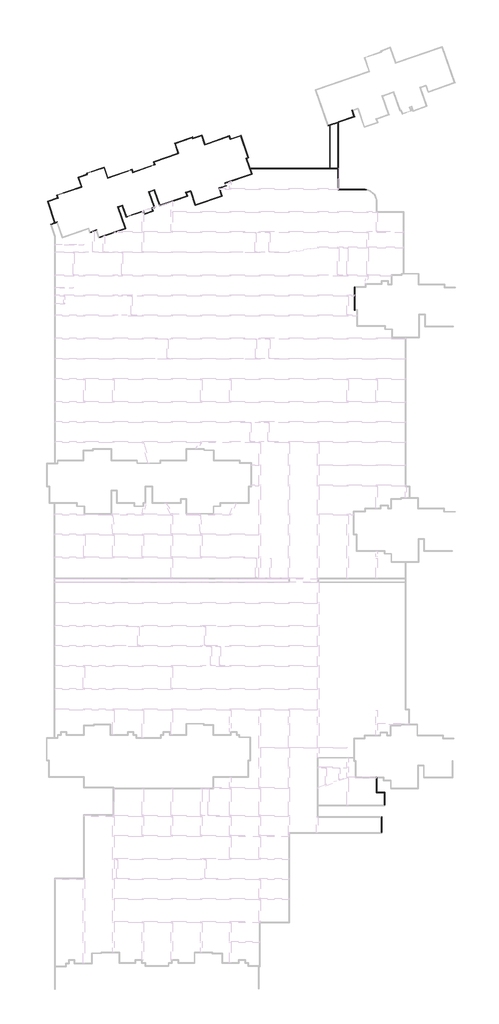
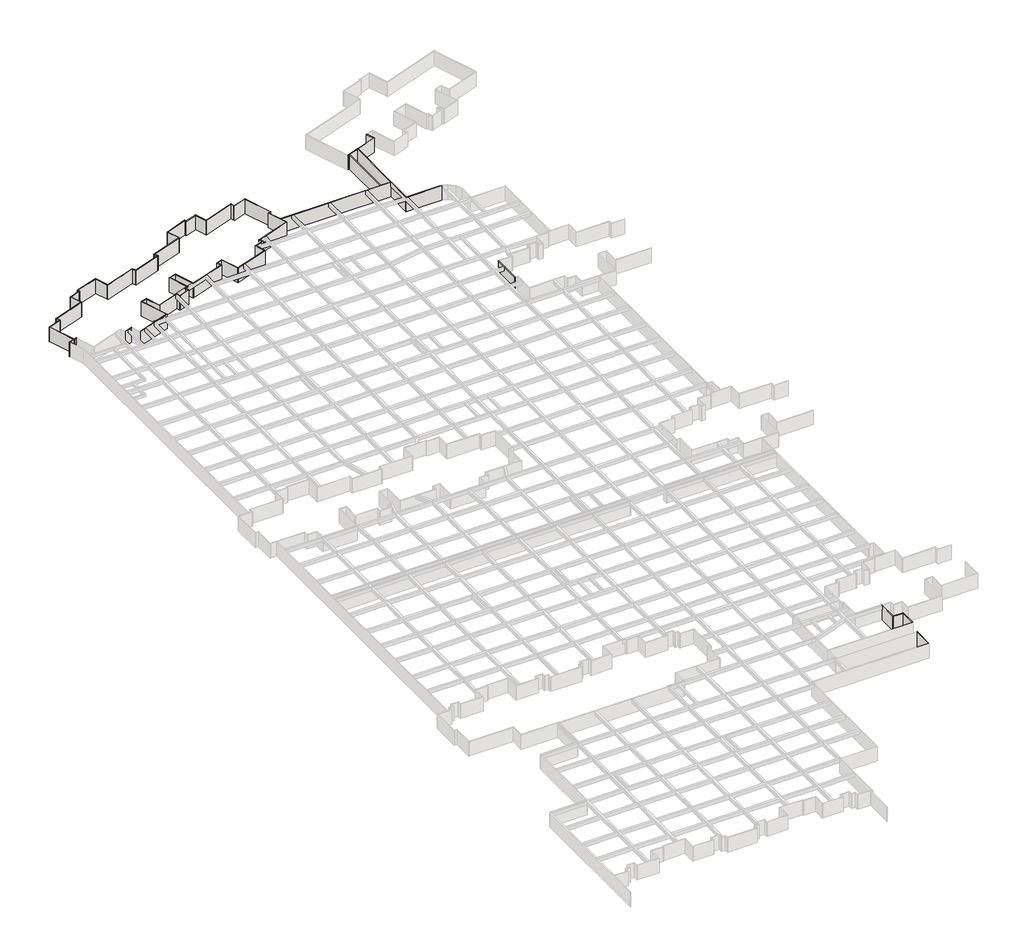
# One storey, part 4 of 14: 62 walls.
"""IFC4 building model written with IfcOpenShell, lengths in millimetres."""

from ifc_helpers import new_model, si_unit, origin, place, context, project, spatial, faceted_brep, element, save

model = new_model("IFC4")

# Units and contexts
model_context = context("Model", 3, world=origin())
ifc_project = project(units=[si_unit("LENGTHUNIT", "METRE", prefix="MILLI")], contexts=[model_context])

# Site, building, storey
site = spatial("IfcSite", under=ifc_project)
building = spatial("IfcBuilding", under=site)
storey = spatial("IfcBuildingStorey", under=building, Name="户型图", Elevation=0.0)

# Walls
placement = place(None, origin())
element("IfcWall", 1, ObjectType="所有墙体", at=placement, inside=storey, context=model_context, shape_type="Brep", body=[
    faceted_brep([(-587687.3228237, -18726.1128295, 0.0), (-586876.8743145, -21142.8199356, 0.0), (-586838.7202272, -21256.5930536, 0.0), (-586838.7202272, -21256.5930536, 3300.0), (-586876.8743145, -21142.8199356, 3300.0), (-587687.3228237, -18726.1128295, 3300.0), (-587575.1897502, -18683.0689754, 0.0), (-587575.1897502, -18683.0689754, 3300.0), (-586725.0230806, -21218.2131681, 3300.0), (-586725.0230806, -21218.2131681, 0.0)], [[[0, 1, 2, 3, 4, 5]], [[6, 7, 8, 9]], [[2, 1, 0, 6, 9]], [[5, 4, 3, 8, 7]], [[3, 2, 9, 8]], [[0, 5, 7, 6]]]),
])
element("IfcWall", 2, ObjectType="所有墙体", at=placement, inside=storey, context=model_context, shape_type="Brep", body=[
    faceted_brep([(-586876.8743145, -21142.8199356, 0.0), (-593604.0549797, -23413.6634153, 0.0), (-593604.0549797, -23413.6634153, 3300.0), (-586876.8743145, -21142.8199356, 3300.0), (-586838.7202272, -21256.5930536, 0.0), (-586838.7202272, -21256.5930536, 3300.0), (-593451.9782472, -23488.9805279, 3300.0), (-593565.6751698, -23527.3603378, 3300.0), (-593565.6751698, -23527.3603378, 0.0), (-593451.9782472, -23488.9805279, 0.0)], [[[0, 1, 2, 3]], [[4, 5, 6, 7, 8, 9]], [[1, 0, 4, 9, 8]], [[3, 2, 7, 6, 5]], [[0, 3, 5, 4]], [[2, 1, 8, 7]]]),
])
element("IfcWall", 3, ObjectType="所有墙体", at=placement, inside=storey, context=model_context, shape_type="Brep", body=[
    faceted_brep([(-593565.6751698, -23527.3603378, 0.0), (-593332.1963521, -24219.021477, 0.0), (-593293.8165422, -24332.7183995, 0.0), (-593293.8165422, -24332.7183995, 3300.0), (-593332.1963521, -24219.021477, 3300.0), (-593565.6751698, -23527.3603378, 3300.0), (-593451.9782472, -23488.9805279, 0.0), (-593451.9782472, -23488.9805279, 3300.0), (-593180.1196197, -24294.3385896, 3300.0), (-593180.1196197, -24294.3385896, 0.0)], [[[0, 1, 2, 3, 4, 5]], [[6, 7, 8, 9]], [[2, 1, 0, 6, 9]], [[5, 4, 3, 8, 7]], [[0, 5, 7, 6]], [[3, 2, 9, 8]]]),
])
element("IfcWall", 4, ObjectType="所有墙体", at=placement, inside=storey, context=model_context, shape_type="Brep", body=[
    faceted_brep([(-593332.1963521, -24219.021477, 0.0), (-596112.814503, -25157.6537082, 0.0), (-596112.814503, -25157.6537082, 3300.0), (-593332.1963521, -24219.021477, 3300.0), (-593293.8165422, -24332.7183995, 0.0), (-593293.8165422, -24332.7183995, 3300.0), (-595960.7377706, -25232.9708208, 3300.0), (-596074.4346931, -25271.3506307, 3300.0), (-596074.4346931, -25271.3506307, 0.0), (-595960.7377706, -25232.9708208, 0.0)], [[[0, 1, 2, 3]], [[4, 5, 6, 7, 8, 9]], [[1, 0, 4, 9, 8]], [[3, 2, 7, 6, 5]], [[0, 3, 5, 4]], [[2, 1, 8, 7]]]),
])
element("IfcWall", 5, ObjectType="所有墙体", at=placement, inside=storey, context=model_context, shape_type="Brep", body=[
    faceted_brep([(-596074.4346931, -25271.3506307, 0.0), (-594137.7360341, -31008.6556848, 0.0), (-594099.3942841, -31122.2398581, 0.0), (-594099.3942841, -31122.2398581, 3300.0), (-594137.7360341, -31008.6556848, 3300.0), (-596074.4346931, -25271.3506307, 3300.0), (-595960.7377706, -25232.9708208, 0.0), (-595960.7377706, -25232.9708208, 3300.0), (-594024.0010516, -30970.3886242, 3300.0), (-593985.6211661, -31084.0857708, 3300.0), (-593985.6211661, -31084.0857708, 0.0), (-594024.0010516, -30970.3886242, 0.0)], [[[0, 1, 2, 3, 4, 5]], [[6, 7, 8, 9, 10, 11]], [[2, 1, 0, 6, 11, 10]], [[5, 4, 3, 9, 8, 7]], [[0, 5, 7, 6]], [[3, 2, 10, 9]]]),
])
element("IfcWall", 6, ObjectType="所有墙体", at=placement, inside=storey, context=model_context, shape_type="Brep", body=[
    faceted_brep([(-593985.6211661, -31084.0857708, 0.0), (-593530.5298151, -30931.4697976, 0.0), (-593416.7566971, -30893.3157103, 0.0), (-593416.7566971, -30893.3157103, 3300.0), (-593530.5298151, -30931.4697976, 3300.0), (-593985.6211661, -31084.0857708, 3300.0), (-594024.0010516, -30970.3886242, 0.0), (-594024.0010516, -30970.3886242, 3300.0), (-593455.1365827, -30779.6185637, 3300.0), (-593455.1365827, -30779.6185637, 0.0)], [[[0, 1, 2, 3, 4, 5]], [[6, 7, 8, 9]], [[2, 1, 0, 6, 9]], [[5, 4, 3, 8, 7]], [[0, 5, 7, 6]], [[3, 2, 9, 8]]]),
])
element("IfcWall", 7, ObjectType="所有墙体", at=placement, inside=storey, context=model_context, shape_type="Brep", body=[
    faceted_brep([(-584459.5809867, -33672.8456024, 0.0), (-582772.9638867, -33103.5070288, 0.0), (-582659.2669642, -33065.1272189, 0.0), (-582659.2669642, -33065.1272189, 3300.0), (-582772.9638867, -33103.5070288, 3300.0), (-584459.5809867, -33672.8456024, 3300.0), (-584497.735074, -33559.0724844, 0.0), (-584497.735074, -33559.0724844, 3300.0), (-582697.6467741, -32951.4302963, 3300.0), (-582697.6467741, -32951.4302963, 0.0)], [[[0, 1, 2, 3, 4, 5]], [[6, 7, 8, 9]], [[2, 1, 0, 6, 9]], [[5, 4, 3, 8, 7]], [[0, 5, 7, 6]], [[3, 2, 9, 8]]]),
])
element("IfcWall", 8, ObjectType="所有墙体", at=placement, inside=storey, context=model_context, shape_type="Brep", body=[
    faceted_brep([(-581987.6202907, -35054.823363, 0.0), (-574770.6130433, -32618.6328334, 0.0), (-574770.6130433, -32618.6328334, 3300.0), (-581987.6202907, -35054.823363, 3300.0), (-582026.0001006, -34941.1264405, 0.0), (-582026.0001006, -34941.1264405, 3300.0), (-574922.6897757, -32543.3157207, 3300.0), (-574808.9928531, -32504.9359109, 3300.0), (-574808.9928531, -32504.9359109, 0.0), (-574922.6897757, -32543.3157207, 0.0)], [[[0, 1, 2, 3]], [[4, 5, 6, 7, 8, 9]], [[1, 0, 4, 9, 8]], [[3, 2, 7, 6, 5]], [[0, 3, 5, 4]], [[2, 1, 8, 7]]]),
])
element("IfcWall", 9, ObjectType="所有墙体", at=placement, inside=storey, context=model_context, shape_type="Brep", body=[
    faceted_brep([(-574808.9928531, -32504.9359109, 0.0), (-576769.5614763, -26696.91811, 0.0), (-576807.9412862, -26583.2211874, 0.0), (-576807.9412862, -26583.2211874, 3300.0), (-576769.5614763, -26696.91811, 3300.0), (-574808.9928531, -32504.9359109, 3300.0), (-574922.6897757, -32543.3157207, 0.0), (-574922.6897757, -32543.3157207, 3300.0), (-576921.6382087, -26621.6009973, 3300.0), (-576921.6382087, -26621.6009973, 0.0)], [[[0, 1, 2, 3, 4, 5]], [[6, 7, 8, 9]], [[2, 1, 0, 6, 9]], [[5, 4, 3, 8, 7]], [[0, 5, 7, 6]], [[3, 2, 9, 8]]]),
])
element("IfcWall", 10, ObjectType="所有墙体", at=placement, inside=storey, context=model_context, shape_type="Brep", body=[
    faceted_brep([(-576769.5614763, -26696.91811, 0.0), (-575651.541738, -26319.5166463, 0.0), (-575537.8448155, -26281.1368364, 0.0), (-575537.8448155, -26281.1368364, 3300.0), (-575651.541738, -26319.5166463, 3300.0), (-576769.5614763, -26696.91811, 3300.0), (-576807.9412862, -26583.2211874, 0.0), (-576807.9412862, -26583.2211874, 3300.0), (-575576.2246253, -26167.4399139, 3300.0), (-575576.2246253, -26167.4399139, 0.0)], [[[0, 1, 2, 3, 4, 5]], [[6, 7, 8, 9]], [[2, 1, 0, 6, 9]], [[5, 4, 3, 8, 7]], [[0, 5, 7, 6]], [[3, 2, 9, 8]]]),
])
element("IfcWall", 11, ObjectType="所有墙体", at=placement, inside=storey, context=model_context, shape_type="Brep", body=[
    faceted_brep([(-575651.541738, -26319.5166463, 0.0), (-574596.1350237, -29446.0692758, 0.0), (-574596.1350237, -29446.0692758, 3300.0), (-575651.541738, -26319.5166463, 3300.0), (-575537.8448155, -26281.1368364, 0.0), (-575537.8448155, -26281.1368364, 3300.0), (-574520.7417912, -29294.2180419, 3300.0), (-574482.3619057, -29407.9151885, 3300.0), (-574482.3619057, -29407.9151885, 0.0), (-574520.7417912, -29294.2180419, 0.0)], [[[0, 1, 2, 3]], [[4, 5, 6, 7, 8, 9]], [[1, 0, 4, 9, 8]], [[3, 2, 7, 6, 5]], [[0, 3, 5, 4]], [[2, 1, 8, 7]]]),
])
element("IfcWall", 12, ObjectType="所有墙体", at=placement, inside=storey, context=model_context, shape_type="Brep", body=[
    faceted_brep([(-574482.3619057, -29407.9151885, 0.0), (-569950.4085273, -27888.1137818, 0.0), (-569836.6354093, -27849.9596945, 0.0), (-569836.6354093, -27849.9596945, 3300.0), (-569950.4085273, -27888.1137818, 3300.0), (-574482.3619057, -29407.9151885, 3300.0), (-574520.7417912, -29294.2180419, 0.0), (-574520.7417912, -29294.2180419, 3300.0), (-569875.0152948, -27736.2625479, 3300.0), (-569875.0152948, -27736.2625479, 0.0)], [[[0, 1, 2, 3, 4, 5]], [[6, 7, 8, 9]], [[2, 1, 0, 6, 9]], [[5, 4, 3, 8, 7]], [[0, 5, 7, 6]], [[3, 2, 9, 8]]]),
])
element("IfcWall", 13, ObjectType="所有墙体", at=placement, inside=storey, context=model_context, shape_type="Brep", body=[
    faceted_brep([(-569950.4085273, -27888.1137818, 0.0), (-569694.5050683, -28646.2060146, 0.0), (-569694.5050683, -28646.2060146, 3300.0), (-569950.4085273, -27888.1137818, 3300.0), (-569836.6354093, -27849.9596945, 0.0), (-569836.6354093, -27849.9596945, 3300.0), (-569619.1879557, -28494.1292822, 3300.0), (-569580.8081458, -28607.8262047, 3300.0), (-569580.8081458, -28607.8262047, 0.0), (-569619.1879557, -28494.1292822, 0.0)], [[[0, 1, 2, 3]], [[4, 5, 6, 7, 8, 9]], [[1, 0, 4, 9, 8]], [[3, 2, 7, 6, 5]], [[0, 3, 5, 4]], [[2, 1, 8, 7]]]),
])
element("IfcWall", 14, ObjectType="所有墙体", at=placement, inside=storey, context=model_context, shape_type="Brep", body=[
    faceted_brep([(-569580.8081458, -28607.8262047, 0.0), (-567259.5995736, -27824.2733903, 0.0), (-567259.5995736, -27824.2733903, 3300.0), (-569580.8081458, -28607.8262047, 3300.0), (-569619.1879557, -28494.1292822, 0.0), (-569619.1879557, -28494.1292822, 3300.0), (-567411.4508075, -27748.8801578, 3300.0), (-567297.7536609, -27710.5002723, 3300.0), (-567297.7536609, -27710.5002723, 0.0), (-567411.4508075, -27748.8801578, 0.0)], [[[0, 1, 2, 3]], [[4, 5, 6, 7, 8, 9]], [[1, 0, 4, 9, 8]], [[3, 2, 7, 6, 5]], [[0, 3, 5, 4]], [[2, 1, 8, 7]]]),
])
element("IfcWall", 15, ObjectType="所有墙体", at=placement, inside=storey, context=model_context, shape_type="Brep", body=[
    faceted_brep([(-567297.7536609, -27710.5002723, 0.0), (-567513.9596543, -27065.7874317, 0.0), (-567552.1137415, -26952.0143137, 0.0), (-567552.1137415, -26952.0143137, 3300.0), (-567513.9596543, -27065.7874317, 3300.0), (-567297.7536609, -27710.5002723, 3300.0), (-567411.4508075, -27748.8801578, 0.0), (-567411.4508075, -27748.8801578, 3300.0), (-567665.8108881, -26990.3941992, 3300.0), (-567665.8108881, -26990.3941992, 0.0)], [[[0, 1, 2, 3, 4, 5]], [[6, 7, 8, 9]], [[2, 1, 0, 6, 9]], [[5, 4, 3, 8, 7]], [[0, 5, 7, 6]], [[3, 2, 9, 8]]]),
])
element("IfcWall", 16, ObjectType="所有墙体", at=placement, inside=storey, context=model_context, shape_type="Brep", body=[
    faceted_brep([(-567513.9596543, -27065.7874317, 0.0), (-566850.6148569, -26841.8671476, 0.0), (-566850.6148569, -26841.8671476, 2500.0), (-566850.6148569, -26841.8671476, 3300.0), (-567238.9034733, -26972.9387979, 3300.0), (-567513.9596543, -27065.7874317, 3300.0), (-567552.1137415, -26952.0143137, 0.0), (-567552.1137415, -26952.0143137, 3300.0), (-567277.2832832, -26859.2418753, 3300.0), (-567002.6915893, -26766.5500349, 3300.0), (-566888.9946667, -26728.170225, 3300.0), (-566888.9946667, -26728.170225, 0.0), (-567002.6915893, -26766.5500349, 0.0)], [[[0, 1, 2, 3, 4, 5]], [[6, 7, 8, 9, 10, 11, 12]], [[1, 0, 6, 12, 11]], [[5, 4, 3, 10, 9, 8, 7]], [[0, 5, 7, 6]], [[3, 2, 1, 11, 10]]]),
])
element("IfcWall", 17, ObjectType="所有墙体", at=placement, inside=storey, context=model_context, shape_type="Brep", body=[
    faceted_brep([(-566888.9946667, -26728.170225, 0.0), (-568292.9695403, -22569.0140692, 0.0), (-568331.3493502, -22455.3171467, 0.0), (-568331.3493502, -22455.3171467, 3300.0), (-568292.9695403, -22569.0140692, 3300.0), (-566933.7711116, -26595.5238154, 3300.0), (-566888.9946667, -26728.170225, 3300.0), (-567002.6915893, -26766.5500349, 0.0), (-567002.6915893, -26766.5500349, 2500.0), (-567002.6915893, -26766.5500349, 3300.0), (-567047.4680341, -26633.9036253, 3300.0), (-568445.0462727, -22493.6969566, 3300.0), (-568445.0462727, -22493.6969566, 0.0)], [[[0, 1, 2, 3, 4, 5, 6]], [[7, 8, 9, 10, 11, 12]], [[2, 1, 0, 7, 12]], [[6, 5, 4, 3, 11, 10, 9]], [[0, 6, 9, 8, 7]], [[3, 2, 12, 11]]]),
])
element("IfcWall", 18, ObjectType="所有墙体", at=placement, inside=storey, context=model_context, shape_type="Brep", body=[
    faceted_brep([(-568292.9695403, -22569.0140692, 0.0), (-566939.5860305, -22112.1626381, 0.0), (-566825.8891079, -22073.7828282, 0.0), (-566825.8891079, -22073.7828282, 3300.0), (-566939.5860305, -22112.1626381, 3300.0), (-568292.9695403, -22569.0140692, 3300.0), (-568331.3493502, -22455.3171467, 0.0), (-568331.3493502, -22455.3171467, 3300.0), (-566864.2689178, -21960.0859057, 3300.0), (-566864.2689178, -21960.0859057, 0.0)], [[[0, 1, 2, 3, 4, 5]], [[6, 7, 8, 9]], [[2, 1, 0, 6, 9]], [[5, 4, 3, 8, 7]], [[0, 5, 7, 6]], [[3, 2, 9, 8]]]),
])
element("IfcWall", 19, ObjectType="所有墙体", at=placement, inside=storey, context=model_context, shape_type="Brep", body=[
    faceted_brep([(-566939.5860305, -22112.1626381, 0.0), (-565497.231347, -26385.0157164, 0.0), (-565497.231347, -26385.0157164, 2500.0), (-565497.231347, -26385.0157164, 3300.0), (-565580.3876017, -26138.6723843, 3300.0), (-566939.5860305, -22112.1626381, 3300.0), (-566825.8891079, -22073.7828282, 0.0), (-566825.8891079, -22073.7828282, 3300.0), (-565466.6906792, -26100.2925744, 3300.0), (-565421.9142343, -26232.938984, 3300.0), (-565383.5344245, -26346.6359066, 3300.0), (-565383.5344245, -26346.6359066, 0.0), (-565421.9142343, -26232.938984, 0.0)], [[[0, 1, 2, 3, 4, 5]], [[6, 7, 8, 9, 10, 11, 12]], [[1, 0, 6, 12, 11]], [[5, 4, 3, 10, 9, 8, 7]], [[0, 5, 7, 6]], [[3, 2, 1, 11, 10]]]),
])
element("IfcWall", 20, ObjectType="所有墙体", at=placement, inside=storey, context=model_context, shape_type="Brep", body=[
    faceted_brep([(-565383.5344245, -26346.6359066, 0.0), (-557803.7395843, -23787.9819143, 0.0), (-557803.7395843, -23787.9819143, 3300.0), (-562267.6529954, -25294.8313886, 3300.0), (-565383.5344245, -26346.6359066, 3300.0), (-565421.9142343, -26232.938984, 0.0), (-565421.9142343, -26232.938984, 2500.0), (-565421.9142343, -26232.938984, 3300.0), (-561948.5420308, -25060.4590103, 3300.0), (-557955.8163167, -23712.6648016, 3300.0), (-557842.1193942, -23674.2849917, 3300.0), (-557842.1193942, -23674.2849917, 0.0), (-557955.8163167, -23712.6648016, 0.0)], [[[0, 1, 2, 3, 4]], [[5, 6, 7, 8, 9, 10, 11, 12]], [[1, 0, 5, 12, 11]], [[4, 3, 2, 10, 9, 8, 7]], [[0, 4, 7, 6, 5]], [[2, 1, 11, 10]]]),
])
element("IfcWall", 21, ObjectType="所有墙体", at=placement, inside=storey, context=model_context, shape_type="Brep", body=[
    faceted_brep([(-557842.1193942, -23674.2849917, 0.0), (-558142.674733, -22783.9153627, 0.0), (-558181.0545428, -22670.2184401, 0.0), (-558181.0545428, -22670.2184401, 3300.0), (-558142.674733, -22783.9153627, 3300.0), (-557842.1193942, -23674.2849917, 3300.0), (-557955.8163167, -23712.6648016, 0.0), (-557955.8163167, -23712.6648016, 3300.0), (-558294.7514654, -22708.59825, 3300.0), (-558294.7514654, -22708.59825, 0.0)], [[[0, 1, 2, 3, 4, 5]], [[6, 7, 8, 9]], [[2, 1, 0, 6, 9]], [[5, 4, 3, 8, 7]], [[0, 5, 7, 6]], [[3, 2, 9, 8]]]),
])
element("IfcWall", 22, ObjectType="所有墙体", at=placement, inside=storey, context=model_context, shape_type="Brep", body=[
    faceted_brep([(-558142.674733, -22783.9153627, 0.0), (-557024.6549947, -22406.513899, 0.0), (-556910.9580721, -22368.1340892, 0.0), (-556910.9580721, -22368.1340892, 3300.0), (-557024.6549947, -22406.513899, 3300.0), (-558142.674733, -22783.9153627, 3300.0), (-558181.0545428, -22670.2184401, 0.0), (-558181.0545428, -22670.2184401, 3300.0), (-556949.337882, -22254.4371666, 3300.0), (-556949.337882, -22254.4371666, 0.0)], [[[0, 1, 2, 3, 4, 5]], [[6, 7, 8, 9]], [[2, 1, 0, 6, 9]], [[5, 4, 3, 8, 7]], [[0, 5, 7, 6]], [[3, 2, 9, 8]]]),
])
element("IfcWall", 23, ObjectType="所有墙体", at=placement, inside=storey, context=model_context, shape_type="Brep", body=[
    faceted_brep([(-557024.6549947, -22406.513899, 0.0), (-555729.3364152, -26243.7850245, 0.0), (-555729.3364152, -26243.7850245, 3300.0), (-557024.6549947, -22406.513899, 3300.0), (-556910.9580721, -22368.1340892, 0.0), (-556910.9580721, -22368.1340892, 3300.0), (-555654.0193026, -26091.7082921, 3300.0), (-555615.6394927, -26205.4052147, 3300.0), (-555615.6394927, -26205.4052147, 0.0), (-555654.0193026, -26091.7082921, 0.0)], [[[0, 1, 2, 3]], [[4, 5, 6, 7, 8, 9]], [[1, 0, 4, 9, 8]], [[3, 2, 7, 6, 5]], [[0, 3, 5, 4]], [[2, 1, 8, 7]]]),
])
element("IfcWall", 24, ObjectType="所有墙体", at=placement, inside=storey, context=model_context, shape_type="Brep", body=[
    faceted_brep([(-555615.6394927, -26205.4052147, 0.0), (-548320.1997124, -23742.7388084, 0.0), (-548320.1997124, -23742.7388084, 3300.0), (-555615.6394927, -26205.4052147, 3300.0), (-555654.0193026, -26091.7082921, 0.0), (-555654.0193026, -26091.7082921, 3300.0), (-548472.0509462, -23667.3455759, 3300.0), (-548358.3537996, -23628.9656904, 3300.0), (-548358.3537996, -23628.9656904, 0.0), (-548472.0509462, -23667.3455759, 0.0)], [[[0, 1, 2, 3]], [[4, 5, 6, 7, 8, 9]], [[1, 0, 4, 9, 8]], [[3, 2, 7, 6, 5]], [[0, 3, 5, 4]], [[2, 1, 8, 7]]]),
])
element("IfcWall", 25, ObjectType="所有墙体", at=placement, inside=storey, context=model_context, shape_type="Brep", body=[
    faceted_brep([(-548358.3537996, -23628.9656904, 0.0), (-549051.4471083, -21562.204502, 0.0), (-549089.6011204, -21448.4316083, 0.0), (-549089.6011204, -21448.4316083, 3300.0), (-549051.4471083, -21562.204502, 3300.0), (-548358.3537996, -23628.9656904, 3300.0), (-548472.0509462, -23667.3455759, 0.0), (-548472.0509462, -23667.3455759, 3300.0), (-549203.3740141, -21486.5856204, 3300.0), (-549203.3740141, -21486.5856204, 0.0)], [[[0, 1, 2, 3, 4, 5]], [[6, 7, 8, 9]], [[2, 1, 0, 6, 9]], [[5, 4, 3, 8, 7]], [[0, 5, 7, 6]], [[3, 2, 9, 8]]]),
])
element("IfcWall", 26, ObjectType="所有墙体", at=placement, inside=storey, context=model_context, shape_type="Brep", body=[
    faceted_brep([(-549051.4471083, -21562.204502, 0.0), (-547206.8501306, -20943.6144929, 0.0), (-547206.8501306, -20943.6144929, 3300.0), (-549051.4471083, -21562.204502, 3300.0), (-549089.6011204, -21448.4316083, 0.0), (-549089.6011204, -21448.4316083, 3300.0), (-547359.0031341, -20868.0714336, 3300.0), (-547245.2300161, -20829.9173463, 3300.0), (-547245.2300161, -20829.9173463, 0.0), (-547359.0031341, -20868.0714336, 0.0)], [[[0, 1, 2, 3]], [[4, 5, 6, 7, 8, 9]], [[1, 0, 4, 9, 8]], [[3, 2, 7, 6, 5]], [[0, 3, 5, 4]], [[2, 1, 8, 7]]]),
])
element("IfcWall", 27, ObjectType="所有墙体", at=placement, inside=storey, context=model_context, shape_type="Brep", body=[
    faceted_brep([(-547245.2300161, -20829.9173463, 0.0), (-547462.7155297, -20185.6350093, 0.0), (-547501.0954152, -20071.9378627, 0.0), (-547501.0954152, -20071.9378627, 3300.0), (-547462.7155297, -20185.6350093, 3300.0), (-547245.2300161, -20829.9173463, 3300.0), (-547359.0031341, -20868.0714336, 0.0), (-547359.0031341, -20868.0714336, 3300.0), (-547614.8685332, -20110.09195, 3300.0), (-547614.8685332, -20110.09195, 0.0)], [[[0, 1, 2, 3, 4, 5]], [[6, 7, 8, 9]], [[2, 1, 0, 6, 9]], [[5, 4, 3, 8, 7]], [[0, 5, 7, 6]], [[3, 2, 9, 8]]]),
])
element("IfcWall", 28, ObjectType="所有墙体", at=placement, inside=storey, context=model_context, shape_type="Brep", body=[
    faceted_brep([(-547462.7155297, -20185.6350093, 0.0), (-540162.2881783, -17737.419233, 0.0), (-540162.2881783, -17737.419233, 3300.0), (-546092.7261364, -19726.205789, 3300.0), (-546652.3562174, -19913.8790754, 3300.0), (-547462.7155297, -20185.6350093, 3300.0), (-547501.0954152, -20071.9378627, 0.0), (-547501.0954152, -20071.9378627, 3300.0), (-546273.8443347, -19660.3762771, 3300.0), (-546161.9464573, -19622.8510562, 3300.0), (-540314.4411818, -17661.8761737, 3300.0), (-540200.6680638, -17623.7220864, 3300.0), (-540200.6680638, -17623.7220864, 0.0), (-540314.4411818, -17661.8761737, 0.0)], [[[0, 1, 2, 3, 4, 5]], [[6, 7, 8, 9, 10, 11, 12, 13]], [[1, 0, 6, 13, 12]], [[5, 4, 3, 2, 11, 10, 9, 8, 7]], [[0, 5, 7, 6]], [[2, 1, 12, 11]]]),
])
element("IfcWall", 29, ObjectType="所有墙体", at=placement, inside=storey, context=model_context, shape_type="Brep", body=[
    faceted_brep([(-540200.6680638, -17623.7220864, 0.0), (-540674.7033886, -16219.4327531, 0.0), (-540715.2108806, -16099.4327531, 0.0), (-541601.5691837, -13473.6716645, 0.0), (-541639.9489936, -13359.9747419, 0.0), (-541639.9489936, -13359.9747419, 3300.0), (-541601.5691837, -13473.6716645, 3300.0), (-540715.2108806, -16099.4327531, 3300.0), (-540674.7033886, -16219.4327531, 3300.0), (-540200.6680638, -17623.7220864, 3300.0), (-540314.4411818, -17661.8761737, 0.0), (-540314.4411818, -17661.8761737, 3300.0), (-541753.6459161, -13398.3545518, 3300.0), (-541753.6459161, -13398.3545518, 0.0)], [[[0, 1, 2, 3, 4, 5, 6, 7, 8, 9]], [[10, 11, 12, 13]], [[4, 3, 2, 1, 0, 10, 13]], [[9, 8, 7, 6, 5, 12, 11]], [[0, 9, 11, 10]], [[5, 4, 13, 12]]]),
])
element("IfcWall", 30, ObjectType="所有墙体", at=placement, inside=storey, context=model_context, shape_type="Brep", body=[
    faceted_brep([(-541601.5691837, -13473.6716645, 0.0), (-541080.5566606, -13297.7974092, 0.0), (-541080.5566606, -13297.7974092, 3300.0), (-541601.5691837, -13473.6716645, 3300.0), (-541639.9489936, -13359.9747419, 0.0), (-541639.9489936, -13359.9747419, 3300.0), (-541232.4078945, -13222.4041767, 3300.0), (-541118.7107479, -13184.0242912, 3300.0), (-541118.7107479, -13184.0242912, 0.0), (-541232.4078945, -13222.4041767, 0.0)], [[[0, 1, 2, 3]], [[4, 5, 6, 7, 8, 9]], [[1, 0, 4, 9, 8]], [[3, 2, 7, 6, 5]], [[0, 3, 5, 4]], [[2, 1, 8, 7]]]),
])
element("IfcWall", 31, ObjectType="所有墙体", at=placement, inside=storey, context=model_context, shape_type="Brep", body=[
    faceted_brep([(-541118.7107479, -13184.0242912, 0.0), (-543153.553482, -7116.2496714, 0.0), (-543153.553482, -7116.2496714, 3300.0), (-541118.7107479, -13184.0242912, 3300.0), (-541232.4078945, -13222.4041767, 0.0), (-541232.4078945, -13222.4041767, 3300.0), (-543229.1723637, -7268.1765773, 3300.0), (-543267.3263758, -7154.4036835, 3300.0), (-543267.3263758, -7154.4036835, 0.0), (-543229.1723637, -7268.1765773, 0.0)], [[[0, 1, 2, 3]], [[4, 5, 6, 7, 8, 9]], [[1, 0, 4, 9, 8]], [[3, 2, 7, 6, 5]], [[0, 3, 5, 4]], [[2, 1, 8, 7]]]),
])
element("IfcWall", 32, ObjectType="所有墙体", at=placement, inside=storey, context=model_context, shape_type="Brep", body=[
    faceted_brep([(-543267.3263758, -7154.4036835, 0.0), (-546010.696458, -8074.3994032, 0.0), (-546124.4798743, -8112.5569441, 0.0), (-546124.4798743, -8112.5569441, 3300.0), (-546010.696458, -8074.3994032, 3300.0), (-543267.3263758, -7154.4036835, 3300.0), (-543229.1723637, -7268.1765773, 0.0), (-543229.1723637, -7268.1765773, 3300.0), (-546084.7784503, -8225.8109096, 3300.0), (-546084.7784503, -8225.8109096, 0.0)], [[[0, 1, 2, 3, 4, 5]], [[6, 7, 8, 9]], [[2, 1, 0, 6, 9]], [[5, 4, 3, 8, 7]], [[0, 5, 7, 6]], [[3, 2, 9, 8]]]),
])
element("IfcWall", 33, ObjectType="所有墙体", at=placement, inside=storey, context=model_context, shape_type="Brep", body=[
    faceted_brep([(-546010.696458, -8074.3994032, 0.0), (-546308.6977282, -7224.3083454, 0.0), (-546308.6977282, -7224.3083454, 3300.0), (-546010.696458, -8074.3994032, 3300.0), (-546124.4798743, -8112.5569441, 0.0), (-546124.4798743, -8112.5569441, 3300.0), (-546382.2434676, -7377.2495897, 3300.0), (-546421.9412201, -7264.0060979, 3300.0), (-546421.9412201, -7264.0060979, 0.0), (-546382.2434676, -7377.2495897, 0.0)], [[[0, 1, 2, 3]], [[4, 5, 6, 7, 8, 9]], [[1, 0, 4, 9, 8]], [[3, 2, 7, 6, 5]], [[0, 3, 5, 4]], [[2, 1, 8, 7]]]),
])
element("IfcWall", 34, ObjectType="所有墙体", at=placement, inside=storey, context=model_context, shape_type="Brep", body=[
    faceted_brep([(-546421.9412201, -7264.0060979, 0.0), (-553005.0297221, -9571.7220982, 0.0), (-553118.2732139, -9611.4198507, 0.0), (-553118.2732139, -9611.4198507, 3300.0), (-553005.0297221, -9571.7220982, 3300.0), (-546421.9412201, -7264.0060979, 3300.0), (-546382.2434676, -7377.2495897, 0.0), (-546382.2434676, -7377.2495897, 3300.0), (-553078.5754614, -9724.6633426, 3300.0), (-553078.5754614, -9724.6633426, 0.0)], [[[0, 1, 2, 3, 4, 5]], [[6, 7, 8, 9]], [[2, 1, 0, 6, 9]], [[5, 4, 3, 8, 7]], [[0, 5, 7, 6]], [[3, 2, 9, 8]]]),
])
element("IfcWall", 35, ObjectType="所有墙体", at=placement, inside=storey, context=model_context, shape_type="Brep", body=[
    faceted_brep([(-553005.0297221, -9571.7220982, 0.0), (-553880.2530201, -7075.0230118, 0.0), (-553880.2530201, -7075.0230118, 3300.0), (-553005.0297221, -9571.7220982, 3300.0), (-553118.2732139, -9611.4198507, 0.0), (-553118.2732139, -9611.4198507, 3300.0), (-553953.9165267, -7227.6283083, 3300.0), (-553993.6144544, -7114.3843166, 3300.0), (-553993.6144544, -7114.3843166, 0.0), (-553953.9165267, -7227.6283083, 0.0)], [[[0, 1, 2, 3]], [[4, 5, 6, 7, 8, 9]], [[1, 0, 4, 9, 8]], [[3, 2, 7, 6, 5]], [[0, 3, 5, 4]], [[2, 1, 8, 7]]]),
])
element("IfcWall", 36, ObjectType="所有墙体", at=placement, inside=storey, context=model_context, shape_type="Brep", body=[
    faceted_brep([(-553993.6144544, -7114.3843166, 0.0), (-556336.40659, -7927.8475196, 0.0), (-556449.7680243, -7967.2088244, 0.0), (-556449.7680243, -7967.2088244, 3300.0), (-556336.40659, -7927.8475196, 3300.0), (-553993.6144544, -7114.3843166, 3300.0), (-553953.9165267, -7227.6283083, 0.0), (-553953.9165267, -7227.6283083, 3300.0), (-556410.0700966, -8080.4528161, 3300.0), (-556410.0700966, -8080.4528161, 0.0)], [[[0, 1, 2, 3, 4, 5]], [[6, 7, 8, 9]], [[2, 1, 0, 6, 9]], [[5, 4, 3, 8, 7]], [[0, 5, 7, 6]], [[3, 2, 9, 8]]]),
])
element("IfcWall", 37, ObjectType="所有墙体", at=placement, inside=storey, context=model_context, shape_type="Brep", body=[
    faceted_brep([(-556336.40659, -7927.8475196, 0.0), (-556468.7913153, -7550.2012395, 0.0), (-556468.7913153, -7550.2012395, 3300.0), (-556336.40659, -7927.8475196, 3300.0), (-556449.7680243, -7967.2088244, 0.0), (-556449.7680243, -7967.2088244, 3300.0), (-556542.3370547, -7703.1424838, 3300.0), (-556582.0348072, -7589.898992, 3300.0), (-556582.0348072, -7589.898992, 0.0), (-556542.3370547, -7703.1424838, 0.0)], [[[0, 1, 2, 3]], [[4, 5, 6, 7, 8, 9]], [[1, 0, 4, 9, 8]], [[3, 2, 7, 6, 5]], [[0, 3, 5, 4]], [[2, 1, 8, 7]]]),
])
element("IfcWall", 38, ObjectType="所有墙体", at=placement, inside=storey, context=model_context, shape_type="Brep", body=[
    faceted_brep([(-556582.0348072, -7589.898992, 0.0), (-561308.5661575, -9246.7948426, 0.0), (-561308.5661575, -9246.7948426, 3300.0), (-556582.0348072, -7589.898992, 3300.0), (-556542.3370547, -7703.1424838, 0.0), (-556542.3370547, -7703.1424838, 3300.0), (-561156.9326281, -9320.7990043, 3300.0), (-561270.1837588, -9360.4994346, 3300.0), (-561270.1837588, -9360.4994346, 0.0), (-561156.9326281, -9320.7990043, 0.0)], [[[0, 1, 2, 3]], [[4, 5, 6, 7, 8, 9]], [[1, 0, 4, 9, 8]], [[3, 2, 7, 6, 5]], [[0, 3, 5, 4]], [[2, 1, 8, 7]]]),
])
element("IfcWall", 39, ObjectType="所有墙体", at=placement, inside=storey, context=model_context, shape_type="Brep", body=[
    faceted_brep([(-561270.1837588, -9360.4994346, 0.0), (-560381.0540858, -11994.4704707, 0.0), (-560342.6716871, -12108.1750626, 0.0), (-560342.6716871, -12108.1750626, 3300.0), (-560381.0540858, -11994.4704707, 3300.0), (-561270.1837588, -9360.4994346, 3300.0), (-561156.9326281, -9320.7990043, 0.0), (-561156.9326281, -9320.7990043, 3300.0), (-560229.4205564, -12068.4746323, 3300.0), (-560229.4205564, -12068.4746323, 0.0)], [[[0, 1, 2, 3, 4, 5]], [[6, 7, 8, 9]], [[2, 1, 0, 6, 9]], [[5, 4, 3, 8, 7]], [[0, 5, 7, 6]], [[3, 2, 9, 8]]]),
])
element("IfcWall", 40, ObjectType="所有墙体", at=placement, inside=storey, context=model_context, shape_type="Brep", body=[
    faceted_brep([(-560381.0540858, -11994.4704707, 0.0), (-567081.9478776, -14343.4833717, 0.0), (-567081.9478776, -14343.4833717, 3300.0), (-560381.0540858, -11994.4704707, 3300.0), (-560342.6716871, -12108.1750626, 0.0), (-560342.6716871, -12108.1750626, 3300.0), (-566929.0066333, -14417.0291111, 3300.0), (-567042.2501251, -14456.7268636, 3300.0), (-567042.2501251, -14456.7268636, 0.0), (-566929.0066333, -14417.0291111, 0.0)], [[[0, 1, 2, 3]], [[4, 5, 6, 7, 8, 9]], [[1, 0, 4, 9, 8]], [[3, 2, 7, 6, 5]], [[0, 3, 5, 4]], [[2, 1, 8, 7]]]),
])
element("IfcWall", 41, ObjectType="所有墙体", at=placement, inside=storey, context=model_context, shape_type="Brep", body=[
    faceted_brep([(-567042.2501251, -14456.7268636, 0.0), (-566821.6264887, -15086.0872024, 0.0), (-566781.9287362, -15199.3306943, 0.0), (-566781.9287362, -15199.3306943, 3300.0), (-566821.6264887, -15086.0872024, 3300.0), (-567042.2501251, -14456.7268636, 3300.0), (-566929.0066333, -14417.0291111, 0.0), (-566929.0066333, -14417.0291111, 3300.0), (-566668.6852444, -15159.6329418, 3300.0), (-566668.6852444, -15159.6329418, 0.0)], [[[0, 1, 2, 3, 4, 5]], [[6, 7, 8, 9]], [[2, 1, 0, 6, 9]], [[5, 4, 3, 8, 7]], [[0, 5, 7, 6]], [[3, 2, 9, 8]]]),
])
element("IfcWall", 42, ObjectType="所有墙体", at=placement, inside=storey, context=model_context, shape_type="Brep", body=[
    faceted_brep([(-566821.6264887, -15086.0872024, 0.0), (-572710.332835, -17150.386027, 0.0), (-572823.5763268, -17190.0837795, 0.0), (-572823.5763268, -17190.0837795, 3300.0), (-572710.332835, -17150.386027, 3300.0), (-566821.6264887, -15086.0872024, 3300.0), (-566781.9287362, -15199.3306943, 0.0), (-566781.9287362, -15199.3306943, 3300.0), (-572783.8785743, -17303.3272713, 3300.0), (-572783.8785743, -17303.3272713, 0.0)], [[[0, 1, 2, 3, 4, 5]], [[6, 7, 8, 9]], [[2, 1, 0, 6, 9]], [[5, 4, 3, 8, 7]], [[0, 5, 7, 6]], [[3, 2, 9, 8]]]),
])
element("IfcWall", 43, ObjectType="所有墙体", at=placement, inside=storey, context=model_context, shape_type="Brep", body=[
    faceted_brep([(-572710.332835, -17150.386027, 0.0), (-572970.4250127, -16408.4360537, 0.0), (-572970.4250127, -16408.4360537, 3300.0), (-572710.332835, -17150.386027, 3300.0), (-572823.5763268, -17190.0837795, 0.0), (-572823.5763268, -17190.0837795, 3300.0), (-573044.4291743, -16560.0695832, 3300.0), (-573084.1296047, -16446.8184525, 3300.0), (-573084.1296047, -16446.8184525, 0.0), (-573044.4291743, -16560.0695832, 0.0)], [[[0, 1, 2, 3]], [[4, 5, 6, 7, 8, 9]], [[1, 0, 4, 9, 8]], [[3, 2, 7, 6, 5]], [[0, 3, 5, 4]], [[2, 1, 8, 7]]]),
])
element("IfcWall", 44, ObjectType="所有墙体", at=placement, inside=storey, context=model_context, shape_type="Brep", body=[
    faceted_brep([(-573084.1296047, -16446.8184525, 0.0), (-579602.0890177, -18647.0366971, 0.0), (-579715.7859402, -18685.416507, 0.0), (-579715.7859402, -18685.416507, 3300.0), (-579602.0890177, -18647.0366971, 3300.0), (-573084.1296047, -16446.8184525, 3300.0), (-573044.4291743, -16560.0695832, 0.0), (-573044.4291743, -16560.0695832, 3300.0), (-579677.4061303, -18799.1134295, 3300.0), (-579677.4061303, -18799.1134295, 0.0)], [[[0, 1, 2, 3, 4, 5]], [[6, 7, 8, 9]], [[2, 1, 0, 6, 9]], [[5, 4, 3, 8, 7]], [[0, 5, 7, 6]], [[3, 2, 9, 8]]]),
])
element("IfcWall", 45, ObjectType="所有墙体", at=placement, inside=storey, context=model_context, shape_type="Brep", body=[
    faceted_brep([(-579602.0890177, -18647.0366971, 0.0), (-580573.3836799, -15769.6588724, 0.0), (-580573.3836799, -15769.6588724, 3300.0), (-579602.0890177, -18647.0366971, 3300.0), (-579715.7859402, -18685.416507, 0.0), (-579715.7859402, -18685.416507, 3300.0), (-580648.7769124, -15921.5101063, 3300.0), (-580687.1567979, -15807.8129597, 3300.0), (-580687.1567979, -15807.8129597, 0.0), (-580648.7769124, -15921.5101063, 0.0)], [[[0, 1, 2, 3]], [[4, 5, 6, 7, 8, 9]], [[1, 0, 4, 9, 8]], [[3, 2, 7, 6, 5]], [[0, 3, 5, 4]], [[2, 1, 8, 7]]]),
])
element("IfcWall", 46, ObjectType="所有墙体", at=placement, inside=storey, context=model_context, shape_type="Brep", body=[
    faceted_brep([(-580687.1567979, -15807.8129597, 0.0), (-585465.5052882, -17410.2435566, 0.0), (-585465.5052882, -17410.2435566, 3300.0), (-580687.1567979, -15807.8129597, 3300.0), (-580648.7769124, -15921.5101063, 0.0), (-580648.7769124, -15921.5101063, 3300.0), (-585313.5783823, -17485.8624383, 3300.0), (-585427.3512761, -17524.0164504, 3300.0), (-585427.3512761, -17524.0164504, 0.0), (-585313.5783823, -17485.8624383, 0.0)], [[[0, 1, 2, 3]], [[4, 5, 6, 7, 8, 9]], [[1, 0, 4, 9, 8]], [[3, 2, 7, 6, 5]], [[0, 3, 5, 4]], [[2, 1, 8, 7]]]),
])
element("IfcWall", 47, ObjectType="所有墙体", at=placement, inside=storey, context=model_context, shape_type="Brep", body=[
    faceted_brep([(-585427.3512761, -17524.0164504, 0.0), (-585366.1363894, -17706.5554395, 0.0), (-585327.9471547, -17820.433365, 0.0), (-585327.9471547, -17820.433365, 3300.0), (-585366.1363894, -17706.5554395, 3300.0), (-585427.3512761, -17524.0164504, 3300.0), (-585313.5783823, -17485.8624383, 0.0), (-585313.5783823, -17485.8624383, 3300.0), (-585215.8140811, -17777.389511, 3300.0), (-585215.8140811, -17777.389511, 0.0)], [[[0, 1, 2, 3, 4, 5]], [[6, 7, 8, 9]], [[2, 1, 0, 6, 9]], [[5, 4, 3, 8, 7]], [[0, 5, 7, 6]], [[3, 2, 9, 8]]]),
])
element("IfcWall", 48, ObjectType="所有墙体", at=placement, inside=storey, context=model_context, shape_type="Brep", body=[
    faceted_brep([(-585366.1363894, -17706.5554395, 0.0), (-587725.5120585, -18612.234904, 0.0), (-587725.5120585, -18612.234904, 3300.0), (-585366.1363894, -17706.5554395, 3300.0), (-585327.9471547, -17820.433365, 0.0), (-585327.9471547, -17820.433365, 3300.0), (-587575.1897502, -18683.0689754, 3300.0), (-587687.3228237, -18726.1128295, 3300.0), (-587687.3228237, -18726.1128295, 0.0), (-587575.1897502, -18683.0689754, 0.0)], [[[0, 1, 2, 3]], [[4, 5, 6, 7, 8, 9]], [[1, 0, 4, 9, 8]], [[3, 2, 7, 6, 5]], [[0, 3, 5, 4]], [[2, 1, 8, 7]]]),
])
element("IfcWall", 49, ObjectType="所有墙体", at=placement, inside=storey, context=model_context, shape_type="Brep", body=[
    faceted_brep([(-594137.7360341, -31008.6556848, 0.0), (-595274.7052593, -31392.4537839, 0.0), (-595274.7052593, -31392.4537839, 3300.0), (-594137.7360341, -31008.6556848, 3300.0), (-594099.3562242, -31122.3526074, 0.0), (-594099.3562242, -31122.3526074, 3300.0), (-595122.6285269, -31467.7708966, 3300.0), (-595236.3254494, -31506.1507065, 3300.0), (-595236.3254494, -31506.1507065, 0.0), (-595122.6285269, -31467.7708966, 0.0)], [[[0, 1, 2, 3]], [[4, 5, 6, 7, 8, 9]], [[1, 0, 4, 9, 8]], [[3, 2, 7, 6, 5]], [[0, 3, 5, 4]], [[2, 1, 8, 7]]]),
])
element("IfcWall", 50, ObjectType="所有墙体", at=placement, inside=storey, context=model_context, shape_type="Brep", body=[
    faceted_brep([(-504707.6529953, -197730.9174567, 0.0), (-504707.6529953, -193330.9174567, 0.0), (-504707.6529953, -193330.9174567, 3300.0), (-504707.6529953, -197730.9174567, 3300.0), (-504827.6529953, -197730.9174567, 0.0), (-504827.6529953, -197730.9174567, 3300.0), (-504827.6529953, -193450.9174567, 3300.0), (-504827.6529953, -193330.9174567, 3300.0), (-504827.6529953, -193330.9174567, 0.0), (-504827.6529953, -193450.9174567, 0.0)], [[[0, 1, 2, 3]], [[4, 5, 6, 7, 8, 9]], [[1, 0, 4, 9, 8]], [[3, 2, 7, 6, 5]], [[0, 3, 5, 4]], [[2, 1, 8, 7]]]),
])
element("IfcWall", 51, ObjectType="所有墙体", at=placement, inside=storey, context=model_context, shape_type="Brep", body=[
    faceted_brep([(-503834.8997281, -190230.9174567, 0.0), (-503834.8997281, -186672.8327534, 0.0), (-503834.8997281, -186672.8327534, 3300.0), (-503834.8997281, -190230.9174567, 3300.0), (-503954.8997281, -190230.9174567, 0.0), (-503954.8997281, -190230.9174567, 3300.0), (-503954.8997281, -186792.8327534, 3300.0), (-503954.8997281, -186672.8327534, 3300.0), (-503954.8997281, -186672.8327534, 0.0), (-503954.8997281, -186792.8327534, 0.0)], [[[0, 1, 2, 3]], [[4, 5, 6, 7, 8, 9]], [[1, 0, 4, 9, 8]], [[3, 2, 7, 6, 5]], [[0, 3, 5, 4]], [[2, 1, 8, 7]]]),
])
element("IfcWall", 52, ObjectType="所有墙体", at=placement, inside=storey, context=model_context, shape_type="Brep", body=[
    faceted_brep([(-503954.8997281, -186672.8327534, 0.0), (-506007.6529952, -186672.8327534, 0.0), (-506127.6529952, -186672.8327534, 0.0), (-506127.6529952, -186672.8327534, 3300.0), (-506007.6529952, -186672.8327534, 3300.0), (-503954.8997281, -186672.8327534, 3300.0), (-503954.8997281, -186792.8327534, 0.0), (-503954.8997281, -186792.8327534, 3300.0), (-506127.6529952, -186792.8327534, 3300.0), (-506127.6529952, -186792.8327534, 0.0)], [[[0, 1, 2, 3, 4, 5]], [[6, 7, 8, 9]], [[2, 1, 0, 6, 9]], [[5, 4, 3, 8, 7]], [[0, 5, 7, 6]], [[3, 2, 9, 8]]]),
])
element("IfcWall", 53, ObjectType="所有墙体", at=placement, inside=storey, context=model_context, shape_type="Brep", body=[
    faceted_brep([(-506007.6529952, -186672.8327534, 0.0), (-506007.6529952, -182584.2232736, 0.0), (-506007.6529952, -182464.2232736, 0.0), (-506007.6529952, -182464.2232736, 3300.0), (-506007.6529952, -182584.2232736, 3300.0), (-506007.6529952, -186672.8327534, 3300.0), (-506127.6529952, -186672.8327534, 0.0), (-506127.6529952, -186672.8327534, 3300.0), (-506127.6529952, -182464.2232736, 3300.0), (-506127.6529952, -182464.2232736, 0.0)], [[[0, 1, 2, 3, 4, 5]], [[6, 7, 8, 9]], [[2, 1, 0, 6, 9]], [[5, 4, 3, 8, 7]], [[0, 5, 7, 6]], [[3, 2, 9, 8]]]),
])
element("IfcWall", 54, ObjectType="所有墙体", at=placement, inside=storey, context=model_context, shape_type="Brep", body=[
    faceted_brep([(-512115.1621146, -48662.2511208, 0.0), (-512115.1621146, -54862.2511208, 0.0), (-512115.1621146, -54862.2511208, 3300.0), (-512115.1621146, -48662.2511208, 3300.0), (-511995.1621146, -48662.2511208, 0.0), (-511995.1621146, -48662.2511208, 3300.0), (-511995.1621146, -54742.2511208, 3300.0), (-511995.1621146, -54862.2511208, 3300.0), (-511995.1621146, -54862.2511208, 0.0), (-511995.1621146, -54742.2511208, 0.0)], [[[0, 1, 2, 3]], [[4, 5, 6, 7, 8, 9]], [[1, 0, 4, 9, 8]], [[3, 2, 7, 6, 5]], [[0, 3, 5, 4]], [[2, 1, 8, 7]]]),
])
element("IfcWall", 55, ObjectType="所有墙体", at=placement, inside=storey, context=model_context, shape_type="Brep", body=[
    faceted_brep([(-509240.5804015, -21839.2569935, 0.0), (-516557.6529954, -21839.2569935, 0.0), (-516677.6529954, -21839.2569935, 0.0), (-516677.6529954, -21839.2569935, 3300.0), (-516557.6529954, -21839.2569935, 3300.0), (-516417.6529954, -21839.2569935, 3300.0), (-509240.5804015, -21839.2569935, 3300.0), (-508928.8010117, -21959.2569935, 0.0), (-508928.8010117, -21959.2569935, 3300.0), (-516417.6529954, -21959.2569935, 3300.0), (-516557.6529954, -21959.2569935, 3300.0), (-516677.6529954, -21959.2569935, 3300.0), (-516677.6529954, -21959.2569935, 2500.0), (-516677.6529954, -21959.2569935, 0.0)], [[[0, 1, 2, 3, 4, 5, 6]], [[7, 8, 9, 10, 11, 12, 13]], [[2, 1, 0, 7, 13]], [[6, 5, 4, 3, 11, 10, 9, 8]], [[0, 6, 8, 7]], [[3, 2, 13, 12, 11]]]),
])
element("IfcWall", 56, ObjectType="所有墙体", at=placement, inside=storey, context=model_context, shape_type="Brep", body=[
    faceted_brep([(-516557.6529954, -21839.2569935, 0.0), (-516557.6529954, -3585.9041026, 0.0), (-516557.6529954, -3458.8762148, 0.0), (-516557.6529954, -3458.8762148, 3300.0), (-516557.6529954, -3585.9041026, 3300.0), (-516557.6529954, -16159.4327531, 3300.0), (-516557.6529954, -21839.2569935, 3300.0), (-516557.6529954, -21839.2569935, 2500.0), (-516677.6529954, -21839.2569935, 0.0), (-516677.6529954, -21839.2569935, 3300.0), (-516677.6529954, -21559.4327531, 3300.0), (-516677.6529954, -16219.4327531, 3300.0), (-516677.6529954, -16099.4327531, 3300.0), (-516677.6529954, -3620.9650679, 3300.0), (-516677.6529954, -3500.5425594, 3300.0), (-516677.6529954, -3500.5425594, 0.0), (-516677.6529954, -3620.9650679, 0.0), (-516677.6529954, -16099.4327531, 0.0), (-516677.6529954, -16219.4327531, 0.0)], [[[0, 1, 2, 3, 4, 5, 6, 7]], [[8, 9, 10, 11, 12, 13, 14, 15, 16, 17, 18]], [[2, 1, 0, 8, 18, 17, 16, 15]], [[6, 5, 4, 3, 14, 13, 12, 11, 10, 9]], [[0, 7, 6, 9, 8]], [[3, 2, 15, 14]]]),
])
element("IfcWall", 57, ObjectType="所有墙体", at=placement, inside=storey, context=model_context, shape_type="Brep", body=[
    faceted_brep([(-516557.6529954, -3585.9041026, 0.0), (-512101.322048, -2038.5789299, 0.0), (-512101.322048, -2038.5789299, 3300.0), (-516557.6529954, -3585.9041026, 3300.0), (-516557.6529954, -3458.8762148, 0.0), (-516557.6529954, -3458.8762148, 3300.0), (-512254.0441132, -1964.579127, 3300.0), (-512140.6831792, -1925.2179959, 3300.0), (-512140.6831792, -1925.2179959, 0.0), (-512254.0441132, -1964.579127, 0.0)], [[[0, 1, 2, 3]], [[4, 5, 6, 7, 8, 9]], [[1, 0, 4, 9, 8]], [[3, 2, 7, 6, 5]], [[0, 3, 5, 4]], [[2, 1, 8, 7]]]),
])
element("IfcWall", 58, ObjectType="所有墙体", at=placement, inside=storey, context=model_context, shape_type="Brep", body=[
    faceted_brep([(-512140.6831792, -1925.2179959, 0.0), (-512675.4931907, -384.9532556, 0.0), (-512714.8543218, -271.5923217, 0.0), (-512714.8543218, -271.5923217, 3300.0), (-512675.4931907, -384.9532556, 3300.0), (-512140.6831792, -1925.2179959, 3300.0), (-512254.0441132, -1964.579127, 0.0), (-512254.0441132, -1964.579127, 3300.0), (-512828.2152558, -310.9534528, 3300.0), (-512828.2152558, -310.9534528, 0.0)], [[[0, 1, 2, 3, 4, 5]], [[6, 7, 8, 9]], [[2, 1, 0, 6, 9]], [[5, 4, 3, 8, 7]], [[0, 5, 7, 6]], [[3, 2, 9, 8]]]),
])
element("IfcWall", 59, ObjectType="所有墙体", at=placement, inside=storey, context=model_context, shape_type="Brep", body=[
    faceted_brep([(-519265.9846589, -4525.5020109, 0.0), (-518931.8479102, -4404.7897793, 0.0), (-518811.8479102, -4361.4378647, 0.0), (-518811.8479102, -4361.4378647, 3300.0), (-518931.8479102, -4404.7897793, 3300.0), (-519265.9846589, -4525.5020109, 3300.0), (-519305.3488556, -4412.1322481, 0.0), (-519305.3488556, -4412.1322481, 3300.0), (-518811.8479102, -4233.8471578, 3300.0), (-518811.8479102, -4233.8471578, 0.0), (-518811.8479102, -4234.9713524, 0.0), (-518811.8479102, -4234.9713524, 3300.0)], [[[0, 1, 2, 3, 4, 5]], [[6, 7, 8, 9]], [[2, 1, 0, 6, 9, 10]], [[5, 4, 3, 11, 8, 7]], [[0, 5, 7, 6]], [[3, 2, 10, 9, 8, 11]]]),
])
element("IfcWall", 60, ObjectType="所有墙体", at=placement, inside=storey, context=model_context, shape_type="Brep", body=[
    faceted_brep([(-518931.8479102, -4404.7897793, 0.0), (-518931.8479102, -16099.4327531, 0.0), (-518931.8479102, -16099.4327531, 3300.0), (-518931.8479102, -4404.7897793, 3300.0), (-518811.8479102, -4361.4378647, 0.0), (-518811.8479102, -4361.4378647, 3300.0), (-518811.8479102, -4361.9992402, 3300.0), (-518811.8479102, -16099.4327531, 3300.0), (-518811.8479102, -16099.4327531, 0.0), (-518811.8479102, -4361.9992402, 0.0)], [[[0, 1, 2, 3]], [[4, 5, 6, 7, 8, 9]], [[1, 0, 4, 9, 8]], [[3, 2, 7, 6, 5]], [[0, 3, 5, 4]], [[2, 1, 8, 7]]]),
])
element("IfcWall", 61, ObjectType="所有墙体", at=placement, inside=storey, context=model_context, shape_type="Brep", body=[
    faceted_brep([(-516677.6529954, -16099.4327531, 0.0), (-518811.8479102, -16099.4327531, 0.0), (-518931.8479102, -16099.4327531, 0.0), (-540715.2108806, -16099.4327531, 0.0), (-540715.2108806, -16099.4327531, 3300.0), (-518931.8479102, -16099.4327531, 3300.0), (-518811.8479102, -16099.4327531, 3300.0), (-516677.6529954, -16099.4327531, 3300.0), (-516677.6529954, -16219.4327531, 0.0), (-516677.6529954, -16219.4327531, 3300.0), (-540674.7033886, -16219.4327531, 3300.0), (-540674.7033886, -16219.4327531, 0.0)], [[[0, 1, 2, 3, 4, 5, 6, 7]], [[8, 9, 10, 11]], [[3, 2, 1, 0, 8, 11]], [[7, 6, 5, 4, 10, 9]], [[4, 3, 11, 10]], [[0, 7, 9, 8]]]),
])
element("IfcWall", 62, ObjectType="所有墙体", at=placement, inside=storey, context=model_context, shape_type="Brep", body=[
    faceted_brep([(-518811.8479102, -4361.9992402, 0.0), (-516677.6529954, -3620.9650679, 0.0), (-516677.6529954, -3620.9650679, 3300.0), (-518811.8479102, -4361.9992402, 3300.0), (-518811.8479102, -4234.9713524, 0.0), (-518811.8479102, -4234.9713524, 3300.0), (-516677.6529954, -3493.9371801, 3300.0), (-516677.6529954, -3493.9371801, 0.0), (-518811.8479102, -4361.4378647, 0.0), (-516677.6529954, -3500.5425594, 0.0), (-516677.6529954, -3500.5425594, 3300.0), (-518811.8479102, -4361.4378647, 3300.0)], [[[0, 1, 2, 3]], [[4, 5, 6, 7]], [[1, 0, 8, 4, 7, 9]], [[3, 2, 10, 6, 5, 11]], [[0, 3, 11, 5, 4, 8]], [[2, 1, 9, 7, 6, 10]]]),
])

save(model, "model.ifc")

# Revit data of these elements
# Type "所有墙体"
#   Layers, outside or top first: 120 mm "默认" (function 1)
# Elements 1, 2, 3, 4, 5, 6, 7, 8, 9, 10, 11, 12, 13, 14, 15, 16, 17, 18, 19, 20, 21, 22, 23, 24, 25, 26, 27, 28, 29, 30, 31, 32, 33, 34, 35, 36, 37, 38, 39, 40, 41, 42, 43, 44, 45, 46, 47, 48, 49, 50, 51, 52, 53, 54, 55, 56, 57, 58, 59, 60, 61, 62 (IfcWall, "所有墙体")
#   Comments = ""
#   Top Offset = 0 mm
#   Base Offset = 0 mm
#   wall height = 3300 mm
#   Phase Created = 新构造
#   Base Constraint = 户型图
#   Top Constraint = 层高
#   Materials on its faces: "默认"
# Materials
#   "默认": class "其他", colour RGB 192 192 192, transparency 0, Cost = 0
